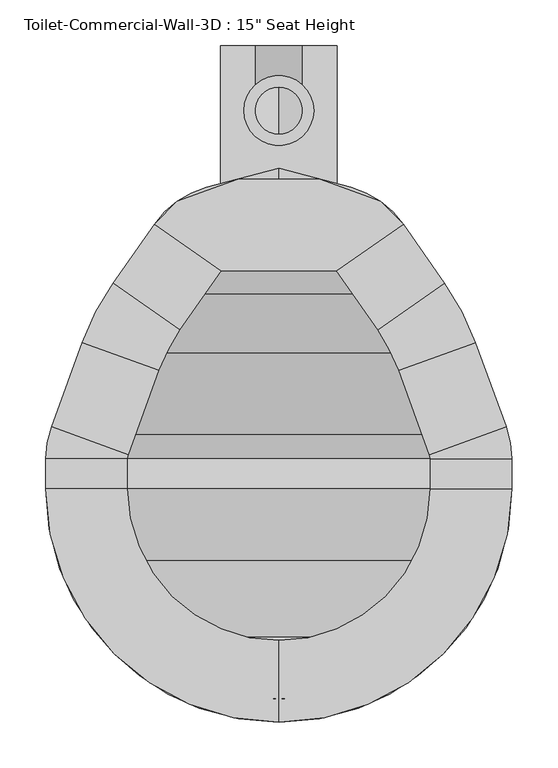
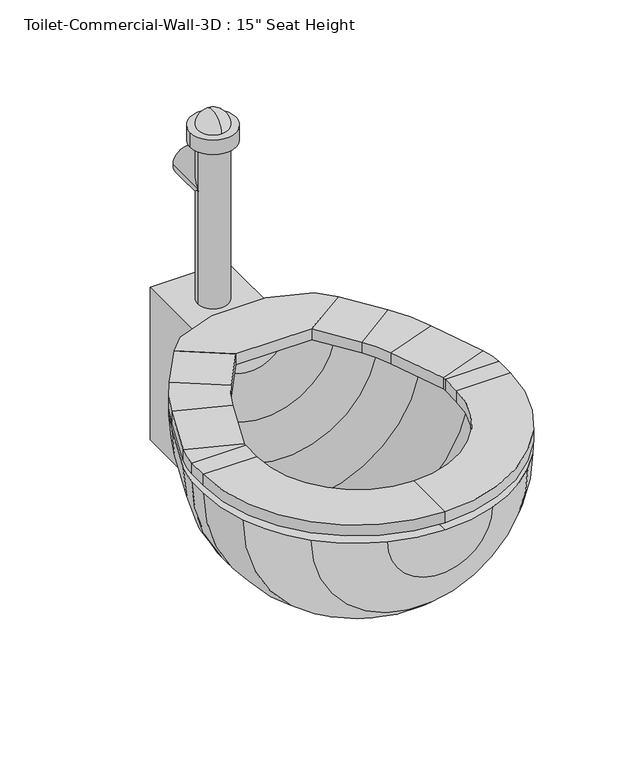
"""IFC4 building model written with IfcOpenShell, lengths in millimetres: flow terminal geometry."""

from ifc_helpers import new_model, si_unit, point, frame, frame_2d, origin, place, context, project, spatial, polyline, circle_curve, ellipse_curve, trimmed, segment, composite_curve, outline, extrude, source, transform, mapped, element, save
from ifc_brep_helpers import plane_surface, cylinder_surface, revolved_surface, advanced_brep


def flow_terminal_62e3d79f(model_context):
    return source(origin(), model_context, "Body", "SolidModel", [
        extrude(outline(polyline([(467.7541169, -443.4722495), (342.0521907, -443.4722495), (269.229574, -392.4813043), (294.1800557, -367.5308226), (360.2423986, -343.4860961), (449.563909, -343.4860961), (515.6262519, -367.5308226), (540.5767337, -392.4813043), (467.7541169, -443.4722495)])), frame((0.0, 0.0, 355.6), z_axis=(0.0, 0.0, 1.0), x_axis=(1.0, 0.0, 0.0)), (0.0, 0.0, 1.0), 19.05),
        advanced_brep(
        [(467.7541169, -443.4722495, 355.6), (467.7541169, -443.4722495, 374.65), (540.5767337, -392.4813043, 374.65), (540.5767337, -392.4813043, 355.6), (585.6810159, -456.8968951, 355.6), (512.8583992, -507.8878403, 355.6), (585.6810159, -456.8968951, 374.65), (512.8583992, -507.8878403, 374.65), (619.360053, -521.5937234, 355.6), (535.821379, -551.9993141, 355.6), (619.360053, -521.5937234, 374.65), (535.821379, -551.9993141, 374.65), (652.7759241, -613.4030747, 355.6), (569.2372501, -643.8086654, 355.6), (652.7759241, -613.4030747, 374.65), (569.2372501, -643.8086654, 374.65), (658.9031538, -648.1523212, 355.6), (570.0031538, -648.1523212, 355.6), (658.9031538, -648.1523212, 374.65), (570.0031538, -648.1523212, 374.65), (658.9031538, -681.0375, 355.6), (570.0031538, -681.0375, 355.6), (658.9031538, -681.0375, 374.65), (570.0031538, -681.0375, 374.65), (404.9031538, -935.0375, 355.6), (404.9031538, -846.1375, 355.6), (404.9031538, -935.0375, 374.65), (404.9031538, -846.1375, 374.65), (150.9031538, -681.0375, 355.6), (239.8031538, -681.0375, 355.6), (150.9031538, -681.0375, 374.65), (239.8031538, -681.0375, 374.65), (150.9031538, -648.1523212, 355.6), (239.8031538, -648.1523212, 355.6), (150.9031538, -648.1523212, 374.65), (239.8031538, -648.1523212, 374.65), (157.0303835, -613.4030747, 355.6), (240.5690575, -643.8086654, 355.6), (157.0303835, -613.4030747, 374.65), (240.5690575, -643.8086654, 374.65), (190.4462546, -521.5937234, 355.6), (273.9849286, -551.9993141, 355.6), (190.4462546, -521.5937234, 374.65), (273.9849286, -551.9993141, 374.65), (224.1252917, -456.8968951, 355.6), (296.9479084, -507.8878403, 355.6), (224.1252917, -456.8968951, 374.65), (296.9479084, -507.8878403, 374.65), (342.0521907, -443.4722495, 355.6), (269.229574, -392.4813043, 355.6), (269.229574, -392.4813043, 374.65), (342.0521907, -443.4722495, 374.65)],
        [
            (0, 1),
            (1, 2),
            (2, 3),
            (3, 0),
            (3, 4),
            (4, 5),
            (5, 0),
            (2, 6),
            (6, 4),
            (1, 7),
            (7, 6),
            (5, 7),
            (8, 9),
            (9, 5, circle_curve(frame((356.8099347, -617.1541514, 355.6), z_axis=(0.0, 0.0, 1.0), x_axis=(0.81915204428899, 0.5735764363510486, 0.0)), 190.5)),
            (4, 8, circle_curve(frame((356.8099347, -617.1541514, 355.6), z_axis=(0.0, 0.0, -1.0), x_axis=(0.81915204428899, 0.5735764363510486, 0.0)), 279.4)),
            (10, 8),
            (6, 10, circle_curve(frame((356.8099347, -617.1541514, 374.65), z_axis=(0.0, 0.0, -1.0), x_axis=(0.81915204428899, 0.5735764363510486, 0.0)), 279.4)),
            (11, 10),
            (7, 11, circle_curve(frame((356.8099347, -617.1541514, 374.65), z_axis=(0.0, 0.0, -1.0), x_axis=(0.81915204428899, 0.5735764363510486, 0.0)), 190.5)),
            (9, 11),
            (8, 12),
            (12, 13),
            (13, 9),
            (10, 14),
            (14, 12),
            (11, 15),
            (15, 14),
            (13, 15),
            (16, 17),
            (17, 13, circle_curve(frame((557.3031538, -648.1523212, 355.6), z_axis=(0.0, 0.0, 1.0), x_axis=(0.9396926207859057, 0.3420201433256761, 0.0)), 12.7)),
            (12, 16, circle_curve(frame((557.3031538, -648.1523212, 355.6), z_axis=(0.0, 0.0, -1.0), x_axis=(0.9396926207859057, 0.3420201433256761, 0.0)), 101.6)),
            (18, 16),
            (14, 18, circle_curve(frame((557.3031538, -648.1523212, 374.65), z_axis=(0.0, 0.0, -1.0), x_axis=(0.9396926207859057, 0.3420201433256761, 0.0)), 101.6)),
            (19, 18),
            (15, 19, circle_curve(frame((557.3031538, -648.1523212, 374.65), z_axis=(0.0, 0.0, -1.0), x_axis=(0.9396926207859057, 0.3420201433256761, 0.0)), 12.7)),
            (17, 19),
            (16, 20),
            (20, 21),
            (21, 17),
            (18, 22),
            (22, 20),
            (19, 23),
            (23, 22),
            (21, 23),
            (24, 25),
            (25, 21, circle_curve(frame((404.9031538, -681.0375, 355.6), z_axis=(0.0, 0.0, 1.0), x_axis=(1.0, 0.0, 0.0)), 165.1)),
            (20, 24, circle_curve(frame((404.9031538, -681.0375, 355.6), z_axis=(0.0, 0.0, -1.0), x_axis=(1.0, 0.0, 0.0)), 254.0)),
            (26, 24),
            (22, 26, circle_curve(frame((404.9031538, -681.0375, 374.65), z_axis=(0.0, 0.0, -1.0), x_axis=(1.0, 0.0, 0.0)), 254.0)),
            (27, 26),
            (23, 27, circle_curve(frame((404.9031538, -681.0375, 374.65), z_axis=(0.0, 0.0, -1.0), x_axis=(1.0, 0.0, 0.0)), 165.1)),
            (25, 27),
            (28, 29),
            (29, 25, circle_curve(frame((404.9031538, -681.0375, 355.6), z_axis=(0.0, 0.0, 1.0), x_axis=(0.0, -1.0, 0.0)), 165.1)),
            (24, 28, circle_curve(frame((404.9031538, -681.0375, 355.6), z_axis=(0.0, 0.0, -1.0), x_axis=(0.0, -1.0, 0.0)), 254.0)),
            (30, 28),
            (26, 30, circle_curve(frame((404.9031538, -681.0375, 374.65), z_axis=(0.0, 0.0, -1.0), x_axis=(0.0, -1.0, 0.0)), 254.0)),
            (31, 30),
            (27, 31, circle_curve(frame((404.9031538, -681.0375, 374.65), z_axis=(0.0, 0.0, -1.0), x_axis=(0.0, -1.0, 0.0)), 165.1)),
            (29, 31),
            (28, 32),
            (32, 33),
            (33, 29),
            (30, 34),
            (34, 32),
            (31, 35),
            (35, 34),
            (33, 35),
            (36, 37),
            (37, 33, circle_curve(frame((252.5031538, -648.1523212, 355.6), z_axis=(0.0, 0.0, 1.0), x_axis=(-1.0, 0.0, 0.0)), 12.7)),
            (32, 36, circle_curve(frame((252.5031538, -648.1523212, 355.6), z_axis=(0.0, 0.0, -1.0), x_axis=(-1.0, 0.0, 0.0)), 101.6)),
            (38, 36),
            (34, 38, circle_curve(frame((252.5031538, -648.1523212, 374.65), z_axis=(0.0, 0.0, -1.0), x_axis=(-1.0, 0.0, 0.0)), 101.6)),
            (39, 38),
            (35, 39, circle_curve(frame((252.5031538, -648.1523212, 374.65), z_axis=(0.0, 0.0, -1.0), x_axis=(-1.0, 0.0, 0.0)), 12.7)),
            (37, 39),
            (36, 40),
            (40, 41),
            (41, 37),
            (38, 42),
            (42, 40),
            (39, 43),
            (43, 42),
            (41, 43),
            (44, 45),
            (45, 41, circle_curve(frame((452.9963729, -617.1541514, 355.6), z_axis=(0.0, 0.0, 1.0), x_axis=(-0.939692620785909, 0.3420201433256672, 0.0)), 190.5)),
            (40, 44, circle_curve(frame((452.9963729, -617.1541514, 355.6), z_axis=(0.0, 0.0, -1.0), x_axis=(-0.939692620785909, 0.3420201433256672, 0.0)), 279.4)),
            (46, 44),
            (42, 46, circle_curve(frame((452.9963729, -617.1541514, 374.65), z_axis=(0.0, 0.0, -1.0), x_axis=(-0.939692620785909, 0.3420201433256672, 0.0)), 279.4)),
            (47, 46),
            (43, 47, circle_curve(frame((452.9963729, -617.1541514, 374.65), z_axis=(0.0, 0.0, -1.0), x_axis=(-0.939692620785909, 0.3420201433256672, 0.0)), 190.5)),
            (45, 47),
            (48, 49),
            (49, 50),
            (50, 51),
            (51, 48),
            (44, 49),
            (48, 45),
            (46, 50),
            (47, 51),
        ],
        [
            plane_surface(frame((540.5767337, -392.4813043, 437.2995365), z_axis=(-0.5735764363510436, 0.8191520442889937, 0.0), x_axis=(0.8191520442889937, 0.5735764363510436, 0.0))),
            plane_surface(frame((467.7541169, -443.4722495, 355.6), z_axis=(0.0, 0.0, -1.0), x_axis=(0.5735764363510436, -0.8191520442889936, 0.0))),
            plane_surface(frame((540.5767337, -392.4813043, 355.6), z_axis=(0.8191520442889944, 0.5735764363510424, 0.0), x_axis=(0.5735764363510424, -0.8191520442889944, 0.0))),
            plane_surface(frame((540.5767337, -392.4813043, 374.65), z_axis=(0.0, 0.0, 1.0), x_axis=(0.573576436351043, -0.819152044288994, 0.0))),
            plane_surface(frame((467.7541169, -443.4722495, 374.65), z_axis=(-0.819152044288994, -0.573576436351043, 0.0), x_axis=(0.573576436351043, -0.819152044288994, 0.0))),
            plane_surface(frame((356.8099347, -617.1541514, 355.6), z_axis=(0.0, 0.0, -1.0), x_axis=(0.81915204428899, 0.5735764363510486, 0.0))),
            cylinder_surface(frame((356.8099347, -617.1541514, 342.9), z_axis=(0.0, 0.0, 1.0), x_axis=(0.81915204428899, 0.5735764363510486, 0.0)), 279.4),
            plane_surface(frame((356.8099347, -617.1541514, 374.65), z_axis=(0.0, 0.0, 1.0), x_axis=(0.81915204428899, 0.5735764363510486, 0.0))),
            revolved_surface(polyline([(512.8583991370526, -507.8878402751253, 374.65), (512.8583991370526, -507.8878402751253, 355.6)]), (356.8099347, -617.1541514, 342.9), (0.0, 0.0, 1.0)),
            plane_surface(frame((535.821379, -551.9993141, 355.6), z_axis=(0.0, 0.0, -1.0000000000000002), x_axis=(0.3420201433256594, -0.9396926207859119, 0.0))),
            plane_surface(frame((619.360053, -521.5937234, 355.6), z_axis=(0.9396926207859121, 0.3420201433256587, 0.0), x_axis=(0.3420201433256587, -0.9396926207859121, 0.0))),
            plane_surface(frame((619.360053, -521.5937234, 374.65), z_axis=(0.0, 0.0, 1.0), x_axis=(0.34202014332565916, -0.9396926207859119, 0.0))),
            plane_surface(frame((535.821379, -551.9993141, 374.65), z_axis=(-0.9396926207859122, -0.34202014332565833, 0.0), x_axis=(0.34202014332565833, -0.9396926207859122, 0.0))),
            plane_surface(frame((557.3031538, -648.1523212, 355.6), z_axis=(0.0, 0.0, -1.0000000000000002), x_axis=(0.9396926207859058, 0.34202014332567615, 0.0))),
            cylinder_surface(frame((557.3031538, -648.1523212, 342.9), z_axis=(0.0, 0.0, 1.0), x_axis=(0.9396926207859057, 0.3420201433256761, 0.0)), 101.6),
            plane_surface(frame((557.3031538, -648.1523212, 374.65), z_axis=(0.0, 0.0, 1.0000000000000002), x_axis=(0.9396926207859058, 0.34202014332567615, 0.0))),
            revolved_surface(polyline([(569.237250083981, -643.8086653797639, 374.65), (569.237250083981, -643.8086653797639, 355.6)]), (557.3031538, -648.1523212, 342.9), (0.0, 0.0, 1.0)),
            plane_surface(frame((570.0031538, -648.1523212, 355.6), z_axis=(0.0, 0.0, -1.0), x_axis=(0.0, -1.0, 0.0))),
            plane_surface(frame((658.9031538, -648.1523212, 355.6), z_axis=(1.0, 0.0, 0.0), x_axis=(0.0, -1.0, 0.0))),
            plane_surface(frame((658.9031538, -648.1523212, 374.65), z_axis=(0.0, 0.0, 1.0), x_axis=(0.0, -1.0, 0.0))),
            plane_surface(frame((570.0031538, -648.1523212, 374.65), z_axis=(-1.0, 0.0, 0.0), x_axis=(0.0, -1.0, 0.0))),
            plane_surface(frame((404.9031538, -681.0375, 355.6), z_axis=(0.0, 0.0, -1.0), x_axis=(1.0, 0.0, 0.0))),
            cylinder_surface(frame((404.9031538, -681.0375, 342.9), z_axis=(0.0, 0.0, 1.0), x_axis=(1.0, 0.0, 0.0)), 254.0),
            plane_surface(frame((404.9031538, -681.0375, 374.65), z_axis=(0.0, 0.0, 1.0), x_axis=(1.0, 0.0, 0.0))),
            revolved_surface(polyline([(570.0031538, -681.0375, 374.65), (570.0031538, -681.0375, 355.6)]), (404.9031538, -681.0375, 342.9), (0.0, 0.0, 1.0)),
            plane_surface(frame((404.9031538, -681.0375, 355.6), z_axis=(0.0, 0.0, -1.0), x_axis=(0.0, -1.0, 0.0))),
            cylinder_surface(frame((404.9031538, -681.0375, 342.9), z_axis=(0.0, 0.0, 1.0), x_axis=(0.0, -1.0, 0.0)), 254.0),
            plane_surface(frame((404.9031538, -681.0375, 374.65), z_axis=(0.0, 0.0, 1.0), x_axis=(0.0, -1.0, 0.0))),
            revolved_surface(polyline([(404.9031538, -846.1375, 374.65), (404.9031538, -846.1375, 355.6)]), (404.9031538, -681.0375, 342.9), (0.0, 0.0, 1.0)),
            plane_surface(frame((239.8031538, -681.0375, 355.6), z_axis=(0.0, 0.0, -1.0), x_axis=(0.0, 1.0, 0.0))),
            plane_surface(frame((150.9031538, -681.0375, 355.6), z_axis=(-1.0, 0.0, 0.0), x_axis=(0.0, 1.0, 0.0))),
            plane_surface(frame((150.9031538, -681.0375, 374.65), z_axis=(0.0, 0.0, 1.0), x_axis=(0.0, 1.0, 0.0))),
            plane_surface(frame((239.8031538, -681.0375, 374.65), z_axis=(1.0, 0.0, 0.0), x_axis=(0.0, 1.0, 0.0))),
            plane_surface(frame((252.5031538, -648.1523212, 355.6), z_axis=(0.0, 0.0, -1.0), x_axis=(-1.0, 0.0, 0.0))),
            cylinder_surface(frame((252.5031538, -648.1523212, 342.9), z_axis=(0.0, 0.0, 1.0), x_axis=(-1.0, 0.0, 0.0)), 101.6),
            plane_surface(frame((252.5031538, -648.1523212, 374.65), z_axis=(0.0, 0.0, 1.0), x_axis=(-1.0, 0.0, 0.0))),
            revolved_surface(polyline([(239.80315380000002, -648.1523212, 374.65), (239.80315380000002, -648.1523212, 355.6)]), (252.5031538, -648.1523212, 342.9), (0.0, 0.0, 1.0)),
            plane_surface(frame((240.5690575, -643.8086654, 355.6), z_axis=(0.0, 0.0, -1.0), x_axis=(0.3420201433256581, 0.9396926207859123, 0.0))),
            plane_surface(frame((157.0303835, -613.4030747, 355.6), z_axis=(-0.9396926207859122, 0.3420201433256583, 0.0), x_axis=(0.3420201433256583, 0.9396926207859122, 0.0))),
            plane_surface(frame((157.0303835, -613.4030747, 374.65), z_axis=(0.0, 0.0, 1.0), x_axis=(0.34202014332565855, 0.9396926207859121, 0.0))),
            plane_surface(frame((240.5690575, -643.8086654, 374.65), z_axis=(0.9396926207859124, -0.3420201433256579, 0.0), x_axis=(0.3420201433256579, 0.9396926207859124, 0.0))),
            plane_surface(frame((452.9963729, -617.1541514, 355.6), z_axis=(0.0, 0.0, -1.0), x_axis=(-0.939692620785909, 0.3420201433256672, 0.0))),
            cylinder_surface(frame((452.9963729, -617.1541514, 342.9), z_axis=(0.0, 0.0, 1.0), x_axis=(-0.939692620785909, 0.3420201433256672, 0.0)), 279.4),
            plane_surface(frame((452.9963729, -617.1541514, 374.65), z_axis=(0.0, 0.0, 1.0), x_axis=(-0.939692620785909, 0.3420201433256672, 0.0))),
            revolved_surface(polyline([(273.98492864028435, -551.9993140964605, 374.65), (273.98492864028435, -551.9993140964605, 355.6)]), (452.9963729, -617.1541514, 342.9), (0.0, 0.0, 1.0)),
            plane_surface(frame((269.229574, -392.4813043, 248.5004635), z_axis=(0.5735764363510469, 0.8191520442889914, 0.0), x_axis=(0.8191520442889914, -0.5735764363510469, 0.0))),
            plane_surface(frame((296.9479084, -507.8878403, 355.6), z_axis=(0.0, 0.0, -1.0), x_axis=(0.5735764363510465, 0.8191520442889916, 0.0))),
            plane_surface(frame((224.1252917, -456.8968951, 355.6), z_axis=(-0.819152044288991, 0.5735764363510473, 0.0), x_axis=(0.5735764363510473, 0.819152044288991, 0.0))),
            plane_surface(frame((224.1252917, -456.8968951, 374.65), z_axis=(0.0, 0.0, 1.0), x_axis=(0.5735764363510473, 0.819152044288991, 0.0))),
            plane_surface(frame((296.9479084, -507.8878403, 374.65), z_axis=(0.8191520442889914, -0.5735764363510468, 0.0), x_axis=(0.5735764363510468, 0.8191520442889914, 0.0))),
        ],
        [
            (0, [[1, 2, 3, 4]]),
            (1, [[5, 6, 7, -4]]),
            (2, [[8, 9, -5, -3]]),
            (3, [[10, 11, -8, -2]]),
            (4, [[-7, 12, -10, -1]]),
            (5, [[13, 14, -6, 15]]),
            (6, [[16, -15, -9, 17]]),
            (7, [[18, -17, -11, 19]]),
            (8, [[20, -19, -12, -14]]),
            (9, [[21, 22, 23, -13]]),
            (10, [[24, 25, -21, -16]]),
            (11, [[26, 27, -24, -18]]),
            (12, [[-23, 28, -26, -20]]),
            (13, [[29, 30, -22, 31]]),
            (14, [[32, -31, -25, 33]]),
            (15, [[34, -33, -27, 35]]),
            (16, [[36, -35, -28, -30]]),
            (17, [[37, 38, 39, -29]]),
            (18, [[40, 41, -37, -32]]),
            (19, [[42, 43, -40, -34]]),
            (20, [[-39, 44, -42, -36]]),
            (21, [[45, 46, -38, 47]]),
            (22, [[48, -47, -41, 49]]),
            (23, [[50, -49, -43, 51]]),
            (24, [[52, -51, -44, -46]]),
            (25, [[53, 54, -45, 55]]),
            (26, [[56, -55, -48, 57]]),
            (27, [[58, -57, -50, 59]]),
            (28, [[60, -59, -52, -54]]),
            (29, [[61, 62, 63, -53]]),
            (30, [[64, 65, -61, -56]]),
            (31, [[66, 67, -64, -58]]),
            (32, [[-63, 68, -66, -60]]),
            (33, [[69, 70, -62, 71]]),
            (34, [[72, -71, -65, 73]]),
            (35, [[74, -73, -67, 75]]),
            (36, [[76, -75, -68, -70]]),
            (37, [[77, 78, 79, -69]]),
            (38, [[80, 81, -77, -72]]),
            (39, [[82, 83, -80, -74]]),
            (40, [[-79, 84, -82, -76]]),
            (41, [[85, 86, -78, 87]]),
            (42, [[88, -87, -81, 89]]),
            (43, [[90, -89, -83, 91]]),
            (44, [[92, -91, -84, -86]]),
            (45, [[93, 94, 95, 96]]),
            (46, [[97, -93, 98, -85]]),
            (47, [[99, -94, -97, -88]]),
            (48, [[100, -95, -99, -90]]),
            (49, [[-98, -96, -100, -92]]),
        ],
    ),
        advanced_brep(
        [(491.7762702, -919.7194257, 342.9), (584.5082762, -860.6426224, 342.9), (643.5850795, -767.9106164, 342.9), (658.9031538, -681.0375, 342.9), (658.9031538, -648.1523212, 342.9), (652.7759241, -613.4030747, 342.9), (619.360053, -521.5937234, 342.9), (585.6810159, -456.8968951, 342.9), (540.5767337, -392.4813043, 342.9), (483.6469009, -352.6186063, 342.9), (404.9031538, -331.5192829, 342.9), (404.9031538, -357.8152978, 342.9), (468.1430637, -374.7603806, 342.9), (525.0728964, -414.6230786, 342.9), (562.9565296, -468.7265139, 342.9), (596.6355667, -533.4233422, 342.9), (628.9077315, -622.0903863, 342.9), (633.5031538, -648.1523212, 342.9), (633.5031538, -681.0375, 342.9), (619.7168869, -759.2233048, 342.9), (566.547764, -842.6821102, 342.9), (483.0889586, -895.8512331, 342.9), (404.9031538, -909.6375, 342.9), (404.9031538, -935.0375, 342.9), (318.0300374, -919.7194257, 342.9), (326.7173491, -895.8512331, 342.9), (243.2585436, -842.6821102, 342.9), (190.0894207, -759.2233048, 342.9), (176.3031538, -681.0375, 342.9), (176.3031538, -648.1523212, 342.9), (180.8985761, -622.0903863, 342.9), (213.1707409, -533.4233422, 342.9), (246.849778, -468.7265139, 342.9), (284.7334112, -414.6230786, 342.9), (341.663244, -374.7603806, 342.9), (326.1594067, -352.6186063, 342.9), (269.229574, -392.4813043, 342.9), (224.1252917, -456.8968951, 342.9), (190.4462546, -521.5937234, 342.9), (157.0303835, -613.4030747, 342.9), (150.9031538, -648.1523212, 342.9), (150.9031538, -681.0375, 342.9), (166.2212281, -767.9106164, 342.9), (225.2980314, -860.6426224, 342.9)],
        [
            (0, 1, circle_curve(frame((404.9031538, -681.0375, 342.9), z_axis=(0.0, 0.0, 1.0), x_axis=(1.0, 0.0, 0.0)), 254.0)),
            (1, 2, circle_curve(frame((404.9031538, -681.0375, 342.9), z_axis=(0.0, 0.0, 1.0), x_axis=(1.0, 0.0, 0.0)), 254.0)),
            (2, 3, circle_curve(frame((404.9031538, -681.0375, 342.9), z_axis=(0.0, 0.0, 1.0), x_axis=(1.0, 0.0, 0.0)), 254.0)),
            (3, 4),
            (4, 5, circle_curve(frame((557.3031538, -648.1523212, 342.9), z_axis=(0.0, 0.0, 1.0), x_axis=(1.0, 0.0, 0.0)), 101.6)),
            (5, 6),
            (6, 7, circle_curve(frame((356.8099347, -617.1541514, 342.9), z_axis=(0.0, 0.0, 1.0), x_axis=(1.0, 0.0, 0.0)), 279.4)),
            (7, 8),
            (8, 9, circle_curve(frame((457.350886, -450.7566703, 342.9), z_axis=(0.0, 0.0, 1.0), x_axis=(1.0, 0.0, 0.0)), 101.6)),
            (9, 10),
            (10, 11),
            (11, 12),
            (12, 13, circle_curve(frame((441.8470487, -472.8984446, 342.9), z_axis=(0.0, 0.0, -1.0), x_axis=(1.0, 0.0, 0.0)), 101.6)),
            (13, 14),
            (14, 15, circle_curve(frame((334.0854485, -628.9837703, 342.9), z_axis=(0.0, 0.0, -1.0), x_axis=(1.0, 0.0, 0.0)), 279.4)),
            (15, 16),
            (16, 17, circle_curve(frame((557.3031538, -648.1523212, 342.9), z_axis=(0.0, 0.0, -1.0), x_axis=(1.0, 0.0, 0.0)), 76.2)),
            (17, 18),
            (18, 19, circle_curve(frame((404.9031538, -681.0375, 342.9), z_axis=(0.0, 0.0, -1.0), x_axis=(1.0, 0.0, 0.0)), 228.6)),
            (19, 20, circle_curve(frame((404.9031538, -681.0375, 342.9), z_axis=(0.0, 0.0, -1.0), x_axis=(1.0, 0.0, 0.0)), 228.6)),
            (20, 21, circle_curve(frame((404.9031538, -681.0375, 342.9), z_axis=(0.0, 0.0, -1.0), x_axis=(1.0, 0.0, 0.0)), 228.6)),
            (21, 22, circle_curve(frame((404.9031538, -681.0375, 342.9), z_axis=(0.0, 0.0, -1.0), x_axis=(1.0, 0.0, 0.0)), 228.6)),
            (22, 23),
            (23, 0, circle_curve(frame((404.9031538, -681.0375, 342.9), z_axis=(0.0, 0.0, 1.0), x_axis=(1.0, 0.0, 0.0)), 254.0)),
            (24, 23, circle_curve(frame((404.9031538, -681.0375, 342.9), z_axis=(0.0, 0.0, 1.0), x_axis=(-1.0, 0.0, 0.0)), 254.0)),
            (22, 25, circle_curve(frame((404.9031538, -681.0375, 342.9), z_axis=(0.0, 0.0, -1.0), x_axis=(-1.0, 0.0, 0.0)), 228.6)),
            (25, 26, circle_curve(frame((404.9031538, -681.0375, 342.9), z_axis=(0.0, 0.0, -1.0), x_axis=(-1.0, 0.0, 0.0)), 228.6)),
            (26, 27, circle_curve(frame((404.9031538, -681.0375, 342.9), z_axis=(0.0, 0.0, -1.0), x_axis=(-1.0, 0.0, 0.0)), 228.6)),
            (27, 28, circle_curve(frame((404.9031538, -681.0375, 342.9), z_axis=(0.0, 0.0, -1.0), x_axis=(-1.0, 0.0, 0.0)), 228.6)),
            (28, 29),
            (29, 30, circle_curve(frame((252.5031538, -648.1523212, 342.9), z_axis=(0.0, 0.0, -1.0), x_axis=(-1.0, 0.0, 0.0)), 76.2)),
            (30, 31),
            (31, 32, circle_curve(frame((475.7208592, -628.9837703, 342.9), z_axis=(0.0, 0.0, -1.0), x_axis=(-1.0, 0.0, 0.0)), 279.4)),
            (32, 33),
            (33, 34, circle_curve(frame((367.9592589, -472.8984446, 342.9), z_axis=(0.0, 0.0, -1.0), x_axis=(-1.0, 0.0, 0.0)), 101.6)),
            (34, 11),
            (10, 35),
            (35, 36, circle_curve(frame((352.4554217, -450.7566703, 342.9), z_axis=(0.0, 0.0, 1.0), x_axis=(-1.0, 0.0, 0.0)), 101.6)),
            (36, 37),
            (37, 38, circle_curve(frame((452.9963729, -617.1541514, 342.9), z_axis=(0.0, 0.0, 1.0), x_axis=(-1.0, 0.0, 0.0)), 279.4)),
            (38, 39),
            (39, 40, circle_curve(frame((252.5031538, -648.1523212, 342.9), z_axis=(0.0, 0.0, 1.0), x_axis=(-1.0, 0.0, 0.0)), 101.6)),
            (40, 41),
            (41, 42, circle_curve(frame((404.9031538, -681.0375, 342.9), z_axis=(0.0, 0.0, 1.0), x_axis=(-1.0, 0.0, 0.0)), 254.0)),
            (42, 43, circle_curve(frame((404.9031538, -681.0375, 342.9), z_axis=(0.0, 0.0, 1.0), x_axis=(-1.0, 0.0, 0.0)), 254.0)),
            (43, 24, circle_curve(frame((404.9031538, -681.0375, 342.9), z_axis=(0.0, 0.0, 1.0), x_axis=(-1.0, 0.0, 0.0)), 254.0)),
            (24, 0, circle_curve(frame((404.9031538, -919.7194257, 342.9), z_axis=(0.0, -1.0, 0.0), x_axis=(1.0, 0.0, 0.0)), 86.8731164)),
            (21, 25, circle_curve(frame((404.9031538, -895.8512331, 342.9), z_axis=(0.0, 1.0, 0.0), x_axis=(1.0, 0.0, 0.0)), 78.1858048)),
            (20, 26, circle_curve(frame((404.9031538, -842.6821102, 342.9), z_axis=(0.0, 1.0, 0.0), x_axis=(1.0, 0.0, 0.0)), 161.6446102)),
            (19, 27, circle_curve(frame((404.9031538, -759.2233048, 342.9), z_axis=(0.0, 1.0, 0.0), x_axis=(1.0, 0.0, 0.0)), 214.8137331)),
            (18, 28, circle_curve(frame((404.9031538, -681.0375, 342.9), z_axis=(0.0, 1.0, 0.0), x_axis=(1.0, 0.0, 0.0)), 228.6)),
            (17, 29, circle_curve(frame((404.9031538, -648.1523212, 342.9), z_axis=(0.0, 1.0, 0.0), x_axis=(1.0, 0.0, 0.0)), 228.6)),
            (16, 30, circle_curve(frame((404.9031538, -622.0903863, 342.9), z_axis=(0.0, 1.0, 0.0), x_axis=(1.0, 0.0, 0.0)), 224.0045777)),
            (15, 31, circle_curve(frame((404.9031538, -533.4233422, 342.9), z_axis=(0.0, 1.0, 0.0), x_axis=(1.0, 0.0, 0.0)), 191.7324129)),
            (14, 32, circle_curve(frame((404.9031538, -468.7265139, 342.9), z_axis=(0.0, 1.0, 0.0), x_axis=(1.0, 0.0, 0.0)), 158.0533758)),
            (13, 33, circle_curve(frame((404.9031538, -414.6230786, 342.9), z_axis=(0.0, 1.0, 0.0), x_axis=(1.0, 0.0, 0.0)), 120.1697426)),
            (12, 34, circle_curve(frame((404.9031538, -374.7603806, 342.9), z_axis=(0.0, 1.0, 0.0), x_axis=(1.0, 0.0, 0.0)), 63.2399099)),
            (9, 35, circle_curve(frame((404.9031538, -352.6186063, 342.9), z_axis=(0.0, 1.0, 0.0), x_axis=(1.0, 0.0, 0.0)), 78.7437471)),
            (8, 36, circle_curve(frame((404.9031538, -392.4813043, 342.9), z_axis=(0.0, 1.0, 0.0), x_axis=(1.0, 0.0, 0.0)), 135.6735798)),
            (7, 37, circle_curve(frame((404.9031538, -456.8968951, 342.9), z_axis=(0.0, 1.0, 0.0), x_axis=(1.0, 0.0, 0.0)), 180.7778621)),
            (6, 38, circle_curve(frame((404.9031538, -521.5937234, 342.9), z_axis=(0.0, 1.0, 0.0), x_axis=(1.0, 0.0, 0.0)), 214.4568992)),
            (5, 39, circle_curve(frame((404.9031538, -613.4030747, 342.9), z_axis=(0.0, 1.0, 0.0), x_axis=(1.0, 0.0, 0.0)), 247.8727703)),
            (4, 40, circle_curve(frame((404.9031538, -648.1523212, 342.9), z_axis=(0.0, 1.0, 0.0), x_axis=(1.0, 0.0, 0.0)), 254.0)),
            (3, 41, circle_curve(frame((404.9031538, -681.0375, 342.9), z_axis=(0.0, 1.0, 0.0), x_axis=(1.0, 0.0, 0.0)), 254.0)),
            (2, 42, circle_curve(frame((404.9031538, -767.9106164, 342.9), z_axis=(0.0, 1.0, 0.0), x_axis=(1.0, 0.0, 0.0)), 238.6819257)),
            (1, 43, circle_curve(frame((404.9031538, -860.6426224, 342.9), z_axis=(0.0, 1.0, 0.0), x_axis=(1.0, 0.0, 0.0)), 179.6051224)),
        ],
        [
            plane_surface(frame((404.9031538, -1040.2477448, 342.9), z_axis=(0.0, 0.0, 1.0), x_axis=(1.0, 0.0, 0.0))),
            plane_surface(frame((404.9031538, -1040.2477448, 342.9), z_axis=(0.0, 0.0, 1.0), x_axis=(-1.0, 0.0, 0.0))),
            revolved_surface(trimmed(ellipse_curve(frame((404.9031538, -681.0375, 342.9), z_axis=(0.0, 0.0, -1.0), x_axis=(1.0, 0.0, 0.0)), 254.0, 254.0), [point((491.7762702, -919.7194257, 342.9))], [point((404.9031538, -935.0375, 342.9))], True, "CARTESIAN"), (404.9031538, -1040.2477448, 342.9), (0.0, -1.0, 0.0)),
            revolved_surface(trimmed(ellipse_curve(frame((404.9031538, -681.0375, 342.9), z_axis=(0.0, 0.0, 1.0), x_axis=(1.0, 0.0, 0.0)), 228.6, 228.6), [point((404.9031538, -909.6375, 342.9))], [point((483.0889586, -895.8512331, 342.9))], True, "CARTESIAN"), (404.9031538, -1040.2477448, 342.9), (0.0, -1.0, 0.0)),
            revolved_surface(trimmed(ellipse_curve(frame((404.9031538, -681.0375, 342.9), z_axis=(0.0, 0.0, 1.0), x_axis=(1.0, 0.0, 0.0)), 228.6, 228.6), [point((483.0889586, -895.8512331, 342.9))], [point((566.547764, -842.6821102, 342.9))], True, "CARTESIAN"), (404.9031538, -1040.2477448, 342.9), (0.0, -1.0, 0.0)),
            revolved_surface(trimmed(ellipse_curve(frame((404.9031538, -681.0375, 342.9), z_axis=(0.0, 0.0, 1.0), x_axis=(1.0, 0.0, 0.0)), 228.6, 228.6), [point((566.547764, -842.6821102, 342.9))], [point((619.7168869, -759.2233048, 342.9))], True, "CARTESIAN"), (404.9031538, -1040.2477448, 342.9), (0.0, -1.0, 0.0)),
            revolved_surface(trimmed(ellipse_curve(frame((404.9031538, -681.0375, 342.9), z_axis=(0.0, 0.0, 1.0), x_axis=(1.0, 0.0, 0.0)), 228.6, 228.6), [point((619.7168869, -759.2233048, 342.9))], [point((633.5031538, -681.0375, 342.9))], True, "CARTESIAN"), (404.9031538, -1040.2477448, 342.9), (0.0, -1.0, 0.0)),
            revolved_surface(polyline([(633.5031538, -681.0375, 342.9), (633.5031538, -648.1523212, 342.9)]), (404.9031538, -1040.2477448, 342.9), (0.0, -1.0, 0.0)),
            revolved_surface(trimmed(ellipse_curve(frame((557.3031538, -648.1523212, 342.9), z_axis=(0.0, 0.0, 1.0), x_axis=(1.0, 0.0, 0.0)), 76.2, 76.2), [point((633.5031538, -648.1523212, 342.9))], [point((628.9077315, -622.0903863, 342.9))], True, "CARTESIAN"), (404.9031538, -1040.2477448, 342.9), (0.0, -1.0, 0.0)),
            revolved_surface(polyline([(628.9077315, -622.0903863, 342.9), (596.6355667, -533.4233422, 342.9)]), (404.9031538, -1040.2477448, 342.9), (0.0, -1.0, 0.0)),
            revolved_surface(trimmed(ellipse_curve(frame((334.0854485, -628.9837703, 342.9), z_axis=(0.0, 0.0, 1.0), x_axis=(1.0, 0.0, 0.0)), 279.4, 279.4), [point((596.6355667, -533.4233422, 342.9))], [point((562.9565296, -468.7265139, 342.9))], True, "CARTESIAN"), (404.9031538, -1040.2477448, 342.9), (0.0, -1.0, 0.0)),
            revolved_surface(polyline([(562.9565296, -468.7265139, 342.9), (525.0728964, -414.6230786, 342.9)]), (404.9031538, -1040.2477448, 342.9), (0.0, -1.0, 0.0)),
            revolved_surface(trimmed(ellipse_curve(frame((441.8470487, -472.8984446, 342.9), z_axis=(0.0, 0.0, 1.0), x_axis=(1.0, 0.0, 0.0)), 101.6, 101.6), [point((525.0728964, -414.6230786, 342.9))], [point((468.1430637, -374.7603806, 342.9))], True, "CARTESIAN"), (404.9031538, -1040.2477448, 342.9), (0.0, -1.0, 0.0)),
            revolved_surface(polyline([(468.1430637, -374.7603806, 342.9), (404.9031538, -357.8152978, 342.9)]), (404.9031538, -1040.2477448, 342.9), (0.0, -1.0, 0.0)),
            revolved_surface(polyline([(404.9031538, -331.5192829, 342.9), (483.6469009, -352.6186063, 342.9)]), (404.9031538, -1040.2477448, 342.9), (0.0, -1.0, 0.0)),
            revolved_surface(trimmed(ellipse_curve(frame((457.350886, -450.7566703, 342.9), z_axis=(0.0, 0.0, -1.0), x_axis=(1.0, 0.0, 0.0)), 101.6, 101.6), [point((483.6469009, -352.6186063, 342.9))], [point((540.5767337, -392.4813043, 342.9))], True, "CARTESIAN"), (404.9031538, -1040.2477448, 342.9), (0.0, -1.0, 0.0)),
            revolved_surface(polyline([(540.5767337, -392.4813043, 342.9), (585.6810159, -456.8968951, 342.9)]), (404.9031538, -1040.2477448, 342.9), (0.0, -1.0, 0.0)),
            revolved_surface(trimmed(ellipse_curve(frame((356.8099347, -617.1541514, 342.9), z_axis=(0.0, 0.0, -1.0), x_axis=(1.0, 0.0, 0.0)), 279.4, 279.4), [point((585.6810159, -456.8968951, 342.9))], [point((619.360053, -521.5937234, 342.9))], True, "CARTESIAN"), (404.9031538, -1040.2477448, 342.9), (0.0, -1.0, 0.0)),
            revolved_surface(polyline([(619.360053, -521.5937234, 342.9), (652.7759241, -613.4030747, 342.9)]), (404.9031538, -1040.2477448, 342.9), (0.0, -1.0, 0.0)),
            revolved_surface(trimmed(ellipse_curve(frame((557.3031538, -648.1523212, 342.9), z_axis=(0.0, 0.0, -1.0), x_axis=(1.0, 0.0, 0.0)), 101.6, 101.6), [point((652.7759241, -613.4030747, 342.9))], [point((658.9031538, -648.1523212, 342.9))], True, "CARTESIAN"), (404.9031538, -1040.2477448, 342.9), (0.0, -1.0, 0.0)),
            cylinder_surface(frame((404.9031538, -1040.2477448, 342.9), z_axis=(0.0, -1.0, 0.0), x_axis=(1.0, 0.0, 0.0)), 254.0),
            revolved_surface(trimmed(ellipse_curve(frame((404.9031538, -681.0375, 342.9), z_axis=(0.0, 0.0, -1.0), x_axis=(1.0, 0.0, 0.0)), 254.0, 254.0), [point((658.9031538, -681.0375, 342.9))], [point((643.5850795, -767.9106164, 342.9))], True, "CARTESIAN"), (404.9031538, -1040.2477448, 342.9), (0.0, -1.0, 0.0)),
            revolved_surface(trimmed(ellipse_curve(frame((404.9031538, -681.0375, 342.9), z_axis=(0.0, 0.0, -1.0), x_axis=(1.0, 0.0, 0.0)), 254.0, 254.0), [point((643.5850795, -767.9106164, 342.9))], [point((584.5082762, -860.6426224, 342.9))], True, "CARTESIAN"), (404.9031538, -1040.2477448, 342.9), (0.0, -1.0, 0.0)),
            revolved_surface(trimmed(ellipse_curve(frame((404.9031538, -681.0375, 342.9), z_axis=(0.0, 0.0, -1.0), x_axis=(1.0, 0.0, 0.0)), 254.0, 254.0), [point((584.5082762, -860.6426224, 342.9))], [point((491.7762702, -919.7194257, 342.9))], True, "CARTESIAN"), (404.9031538, -1040.2477448, 342.9), (0.0, -1.0, 0.0)),
        ],
        [
            (0, [[1, 2, 3, 4, 5, 6, 7, 8, 9, 10, 11, 12, 13, 14, 15, 16, 17, 18, 19, 20, 21, 22, 23, 24]]),
            (1, [[25, -23, 26, 27, 28, 29, 30, 31, 32, 33, 34, 35, 36, -11, 37, 38, 39, 40, 41, 42, 43, 44, 45, 46]]),
            (2, [[-25, 47, -24]]),
            (3, [[-26, -22, 48]]),
            (4, [[-27, -48, -21, 49]]),
            (5, [[-28, -49, -20, 50]]),
            (6, [[-29, -50, -19, 51]]),
            (7, [[-30, -51, -18, 52]]),
            (8, [[-31, -52, -17, 53]]),
            (9, [[-32, -53, -16, 54]]),
            (10, [[-33, -54, -15, 55]]),
            (11, [[-34, -55, -14, 56]]),
            (12, [[-35, -56, -13, 57]]),
            (13, [[-36, -57, -12]]),
            (14, [[-37, -10, 58]]),
            (15, [[-38, -58, -9, 59]]),
            (16, [[-39, -59, -8, 60]]),
            (17, [[-40, -60, -7, 61]]),
            (18, [[-41, -61, -6, 62]]),
            (19, [[-42, -62, -5, 63]]),
            (20, [[-43, -63, -4, 64]]),
            (21, [[-44, -64, -3, 65]]),
            (22, [[-45, -65, -2, 66]]),
            (23, [[-46, -66, -1, -47]]),
        ],
    ),
        advanced_brep(
        [(404.9031538, -243.3551912, 647.7), (404.9031538, -268.9727737, 673.3175826), (404.9031538, -294.5903563, 647.7), (404.9031538, -268.9727737, 647.7)],
        [
            (0, 1, circle_curve(frame((404.9031538, -268.9727737, 647.7), z_axis=(1.0, 0.0, 0.0), x_axis=(0.0, -1.0, 0.0)), 25.6175826)),
            (1, 2, circle_curve(frame((404.9031538, -268.9727737, 647.7), z_axis=(1.0, 0.0, 0.0), x_axis=(0.0, 1.0, 0.0)), 25.6175826)),
            (2, 0, circle_curve(frame((404.9031538, -268.9727737, 647.7), z_axis=(0.0, 0.0, 1.0), x_axis=(0.0, -1.0, 0.0)), 25.6175826)),
            (0, 2, circle_curve(frame((404.9031538, -268.9727737, 647.7), z_axis=(0.0, 0.0, 1.0), x_axis=(0.0, -1.0, 0.0)), 25.6175826)),
            (3, 0),
            (2, 3),
        ],
        [
            revolved_surface(trimmed(ellipse_curve(frame((404.9031538, -268.9727737, 647.7), z_axis=(1.0, 0.0, 0.0), x_axis=(0.0, 1.0, 0.0)), 25.6175826, 25.6175826), [point((404.9031538, -268.9727737, 673.3175826))], [point((404.9031538, -294.5903563, 647.7))], True, "CARTESIAN"), (404.9031538, -268.9727737, 712.3277273), (0.0, 0.0, -1.0)),
            plane_surface(frame((404.9031538, -268.9727737, 647.7), z_axis=(0.0, 0.0, -1.0), x_axis=(0.0, -1.0, 0.0))),
        ],
        [
            (0, [[1, 2, 3]]),
            (0, [[-2, -1, 4]]),
            (1, [[5, -3, 6]]),
            (1, [[-6, -4, -5]]),
        ],
    ),
        extrude(outline(composite_curve([segment(trimmed(circle_curve(frame_2d((404.9031538, -268.9727737)), 38.1), [point((366.8031538, -268.9727737))], [point((443.0031538, -268.9727737))], False, "CARTESIAN"), True, "CONTINUOUS"), segment(trimmed(circle_curve(frame_2d((404.9031538, -268.9727737)), 38.1), [point((443.0031538, -268.9727737))], [point((366.8031538, -268.9727737))], False, "CARTESIAN"), True, "CONTINUOUS")], self_intersect=False)), frame((0.0, 0.0, 622.3), z_axis=(0.0, 0.0, 1.0), x_axis=(1.0, 0.0, 0.0)), (0.0, 0.0, 1.0), 25.4),
        extrude(outline(composite_curve([segment(trimmed(circle_curve(frame_2d((544.2113641, 404.9031538)), 25.4), [point((544.2113641, 379.5031538))], [point((544.2113641, 430.3031538))], False, "CARTESIAN"), True, "CONTINUOUS"), segment(trimmed(circle_curve(frame_2d((544.2113641, 404.9031538)), 25.4), [point((544.2113641, 430.3031538))], [point((544.2113641, 379.5031538))], False, "CARTESIAN"), True, "CONTINUOUS")], self_intersect=False)), frame((0.0, -269.08125, 0.0), z_axis=(0.0, 1.0, 0.0), x_axis=(0.0, 0.0, 1.0)), (0.0, 0.0, 1.0), 70.64375),
        extrude(outline(polyline([(-351.2412941, 342.9), (-198.4375, 342.9), (-198.4375, 76.2), (-418.4829017, 76.2), (-498.9801282, 134.0328588), (-394.9478185, 206.8770663), (-351.2412941, 269.296452), (-351.2412941, 342.9)])), frame((341.4031538, 0.0, 0.0), z_axis=(1.0, 0.0, 0.0), x_axis=(0.0, 1.0, 0.0)), (0.0, 0.0, 1.0), 127.0),
        extrude(outline(composite_curve([segment(trimmed(circle_curve(frame_2d((404.9031538, -268.9727737)), 25.4), [point((379.5031538, -268.9727737))], [point((430.3031538, -268.9727737))], False, "CARTESIAN"), True, "CONTINUOUS"), segment(trimmed(circle_curve(frame_2d((404.9031538, -268.9727737)), 25.4), [point((430.3031538, -268.9727737))], [point((379.5031538, -268.9727737))], False, "CARTESIAN"), True, "CONTINUOUS")], self_intersect=False)), frame((0.0, 0.0, 342.9), z_axis=(0.0, 0.0, 1.0), x_axis=(1.0, 0.0, 0.0)), (0.0, 0.0, 1.0), 279.4),
    ])


if __name__ == "__main__":
    model = new_model("IFC4")
    model_context = context("Model", 3, world=origin())
    ifc_project = project(units=[si_unit("LENGTHUNIT", "METRE", prefix="MILLI")], contexts=[model_context])
    site = spatial("IfcSite", under=ifc_project)
    building = spatial("IfcBuilding", under=site)
    placement = place(None, origin())
    flow_terminal_shape = flow_terminal_62e3d79f(model_context)
    element("IfcFlowTerminal", 1, ObjectType="Toilet-Commercial-Wall-3D : 15\" Seat Height", at=placement, inside=building, context=model_context, shape_type="MappedRepresentation", body=[
        mapped(flow_terminal_shape, transform((0.0, 0.0, 0.0), x_axis=(1.0, 0.0, 0.0), y_axis=(0.0, 1.0, 0.0), z_axis=(0.0, 0.0, 1.0))),
    ])
    save(model, "model.ifc")

# Revit data of these elements
# Type "Toilet-Commercial-Wall-3D : 15\" Seat Height"
#   Assembly Code = "D2010110"
#   Mounting Height = 1' - 3"
#   Piping Material = Metal - Steel, Polished
#   Toilet - Bowl Material = Porcelain - Ivory
#   Toilet - Seat Material = Laminate - Ivory,Matte
#   Default Elevation = 0
# Element 1 (IfcFlowTerminal, "Toilet-Commercial-Wall-3D : 15\" Seat Height")
#   Materials on its faces: "Laminate - Ivory,Matte", "Porcelain - Ivory", "Metal - Steel, Polished"
# Materials
#   "Metal - Steel, Polished": class "Unassigned", colour RGB 57 57 57, transparency 0
#   "Porcelain - Ivory": class "Unassigned", colour RGB 247 247 239, transparency 0
#   "Laminate - Ivory,Matte": class "Unassigned", colour RGB 247 247 239, transparency 0, Description = "Laminate"
